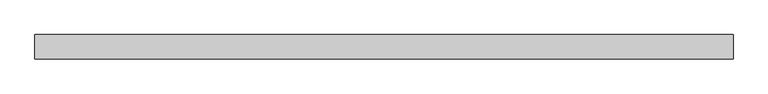
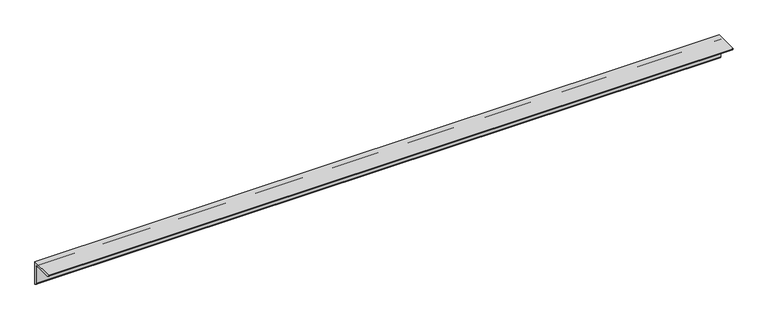
"""IFC4 building model written with IfcOpenShell, lengths in millimetres: member geometry, 0912_Steel Framing_L-KSD3502 : H_SB_AR_S03_L-130x130x12_HBR3."""

from ifc_helpers import new_model, si_unit, point, frame, frame_2d, origin, place, context, project, spatial, polyline, circle_curve, trimmed, segment, composite_curve, outline, extrude, source, transform, mapped, element, save


def member_3c30417d(model_context):
    return source(origin(), model_context, "Body", "SweptSolid", [
        extrude(outline(composite_curve([segment(polyline([(36.4, 36.4), (36.4, -93.6)]), True, "CONTINUOUS"), segment(trimmed(circle_curve(frame_2d((36.4, -81.6)), 12.0), [point((36.4, -93.6))], [point((24.4, -81.6))], False, "CARTESIAN"), True, "CONTINUOUS"), segment(polyline([(24.4, -81.6), (24.4, 12.4)]), True, "CONTINUOUS"), segment(trimmed(circle_curve(frame_2d((12.4, 12.4)), 12.0), [point((24.4, 12.4))], [point((12.4, 24.4))], True, "CARTESIAN"), True, "CONTINUOUS"), segment(polyline([(12.4, 24.4), (-81.6, 24.4)]), True, "CONTINUOUS"), segment(trimmed(circle_curve(frame_2d((-81.6, 36.4)), 12.0), [point((-81.6, 24.4))], [point((-93.6, 36.4))], False, "CARTESIAN"), True, "CONTINUOUS"), segment(polyline([(-93.6, 36.4), (36.4, 36.4)]), True, "CONTINUOUS")], self_intersect=False)), frame((-1825.7683013, 0.0, 0.0), z_axis=(1.0, 0.0, 0.0), x_axis=(0.0, 1.0, 0.0)), (0.0, 0.0, 1.0), 3729.3286027),
    ])


if __name__ == "__main__":
    model = new_model("IFC4")
    model_context = context("Model", 3, world=origin())
    ifc_project = project(units=[si_unit("LENGTHUNIT", "METRE", prefix="MILLI")], contexts=[model_context])
    site = spatial("IfcSite", under=ifc_project)
    building = spatial("IfcBuilding", under=site)
    placement = place(None, origin())
    member_shape = member_3c30417d(model_context)
    element("IfcMember", 1, ObjectType="0912_Steel Framing_L-KSD3502 : H_SB_AR_S03_L-130x130x12_HBR3", at=placement, inside=building, context=model_context, shape_type="MappedRepresentation", body=[
        mapped(member_shape, transform((0.0, 0.0, 0.0), x_axis=(1.0, 0.0, 0.0), y_axis=(0.0, 1.0, 0.0), z_axis=(0.0, 0.0, 1.0))),
    ])
    save(model, "model.ifc")

# Revit data of these elements
# Type "0912_Steel Framing_L-KSD3502 : H_SB_AR_S03_L-130x130x12_HBR3"
#   k = 25 mm
#   Perimeter = 0.52 m²/m
#   Nominal Weight = 23.40 kgf/m
#   Length [instance default] = 1000 mm
#   b = 130 mm
#   d = 130 mm
#   t = 12 mm
#   x = 36.4 mm
#   y = 36.4 mm
#   A = 2976.00 m²
#   Structural Material [instance default] = Steel, 45-345
# Element 1 (IfcMember, "0912_Steel Framing_L-KSD3502 : H_SB_AR_S03_L-130x130x12_HBR3")
#   Structural Material = Steel ASTM A36
#   Materials on its faces: "Steel ASTM A36"
# Materials
#   "Steel, 45-345": class "Metal", colour RGB 189 187 185, transparency 0, Description = "Steel 345 MPa", Cost = 0
#   "Steel ASTM A36": class "Metal", colour RGB 199 199 199, transparency 0, Description = "Structural steel, ASTM A36 Grade B, mill finish", Cost = 0
